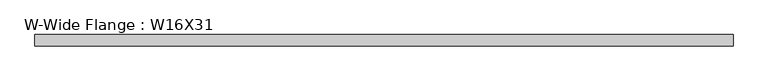
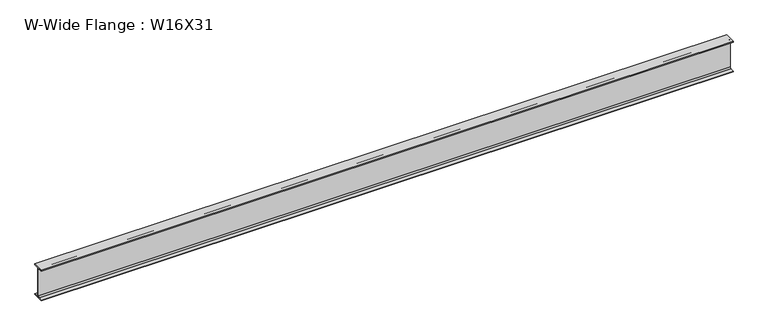
"""IFC4 building model written with IfcOpenShell, lengths in millimetres: beam geometry, W-Wide Flange : W16X31."""

from ifc_helpers import new_model, si_unit, point, frame, frame_2d, origin, place, context, project, spatial, polyline, circle_curve, trimmed, segment, composite_curve, outline, extrude, source, transform, mapped, element, save


def w_wide_flange_w16x31_38feb42c(model_context):
    return source(origin(), model_context, "Body", "SweptSolid", [
        extrude(outline(composite_curve([segment(polyline([(70.231, -190.754), (70.231, -201.93), (-70.231, -201.93), (-70.231, -190.754), (-20.8915, -190.754)]), True, "CONTINUOUS"), segment(trimmed(circle_curve(frame_2d((-20.8915, -173.355)), 17.399), [point((-20.8915, -190.754))], [point((-3.4925, -173.355))], True, "CARTESIAN"), True, "CONTINUOUS"), segment(polyline([(-3.4925, -173.355), (-3.4925, 173.355)]), True, "CONTINUOUS"), segment(trimmed(circle_curve(frame_2d((-20.8915, 173.355)), 17.399), [point((-3.4925, 173.355))], [point((-20.8915, 190.754))], True, "CARTESIAN"), True, "CONTINUOUS"), segment(polyline([(-20.8915, 190.754), (-70.231, 190.754), (-70.231, 201.93), (70.231, 201.93), (70.231, 190.754), (20.8915, 190.754)]), True, "CONTINUOUS"), segment(trimmed(circle_curve(frame_2d((20.8915, 173.355)), 17.399), [point((20.8915, 190.754))], [point((3.4925, 173.355))], True, "CARTESIAN"), True, "CONTINUOUS"), segment(polyline([(3.4925, 173.355), (3.4925, -173.355)]), True, "CONTINUOUS"), segment(trimmed(circle_curve(frame_2d((20.8915, -173.355)), 17.399), [point((3.4925, -173.355))], [point((20.8915, -190.754))], True, "CARTESIAN"), True, "CONTINUOUS"), segment(polyline([(20.8915, -190.754), (70.231, -190.754)]), True, "CONTINUOUS")], self_intersect=False)), frame((-4330.0820758, 0.0, 0.0), z_axis=(1.0, 0.0, 0.0), x_axis=(0.0, 1.0, 0.0)), (0.0, 0.0, 1.0), 8660.1641516),
    ])


if __name__ == "__main__":
    model = new_model("IFC4")
    model_context = context("Model", 3, world=origin())
    ifc_project = project(units=[si_unit("LENGTHUNIT", "METRE", prefix="MILLI")], contexts=[model_context])
    site = spatial("IfcSite", under=ifc_project)
    building = spatial("IfcBuilding", under=site)
    placement = place(None, origin())
    w_wide_flange_w16x31_shape = w_wide_flange_w16x31_38feb42c(model_context)
    element("IfcBeam", 1, ObjectType="W-Wide Flange : W16X31", at=placement, inside=building, context=model_context, shape_type="MappedRepresentation", body=[
        mapped(w_wide_flange_w16x31_shape, transform((0.0, 0.0, 0.0), x_axis=(1.0, 0.0, 0.0), y_axis=(0.0, 1.0, 0.0), z_axis=(0.0, 0.0, 1.0))),
    ])
    save(model, "model.ifc")

# Revit data of these elements
# Type "W-Wide Flange : W16X31"
#   Assembly Code = "B10"
#   W = 31
#   Start Extension Calculation [instance default] = 10' - 0"
#   Start Extension [instance default] = -0' - 0 1/2"
#   End Extension Calculation [instance default] = 10' - 0"
#   End Extension [instance default] = -0' - 0 1/2"
#   Length [instance default] = 5' - 0"
#   bf = 0' - 5.53"
#   d = 1' - 3.9"
#   k = 0' - 1 1/8"
#   k2 = 0' - 0.685"
#   tf = 0' - 0.44"
#   tw = 0' - 0.275"
#   A = 0.0634028 SF
#   Beam Material [instance default] = Metal - Steel - ASTM A992
# Element 1 (IfcBeam, "W-Wide Flange : W16X31")
#   Materials on its faces: "Metal - Steel - ASTM A992"
# Materials
#   "Metal - Steel - ASTM A992": class "Metal", colour RGB 128 0 0, transparency 0
